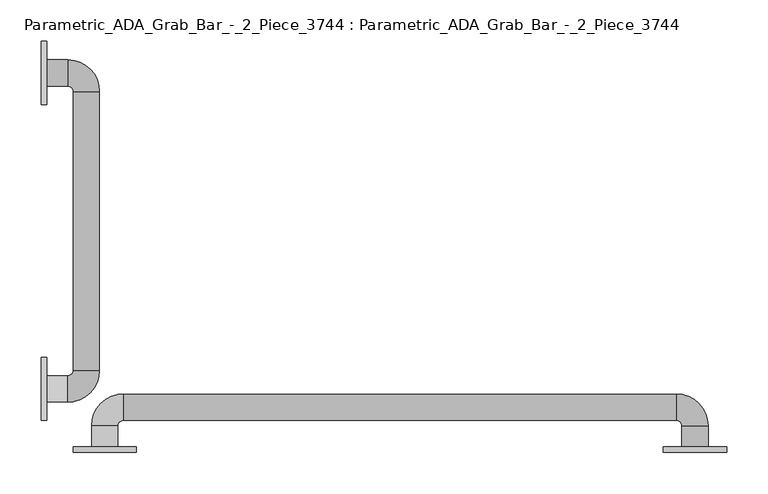
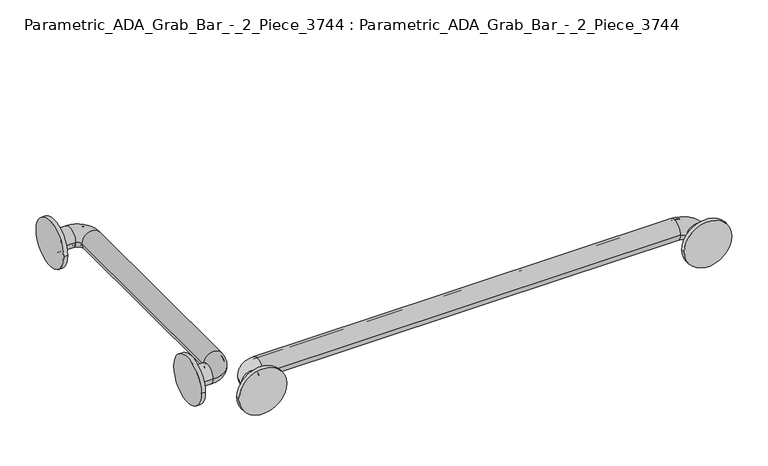
"""IFC4 building model written with IfcOpenShell, lengths in millimetres: proxy geometry, Parametric_ADA_Grab_Bar_-_2_Piece_3744 : Parametric_ADA_Grab_Bar_-_2_Piece_3744."""

from ifc_helpers import new_model, si_unit, point, frame, frame_2d, origin, place, context, project, spatial, polyline, circle_curve, ellipse_curve, trimmed, segment, composite_curve, outline, extrude, source, transform, mapped, element, save
from ifc_brep_helpers import plane_surface, cylinder_surface, revolved_surface, advanced_brep


def parametric_ada_grab_bar_2_piece_3744_parametric_ada_grab_bar_39837210(model_context):
    return source(origin(), model_context, "Body", "SolidModel", [
        advanced_brep(
        [(6.35, 454.81875, 838.2), (6.35, 486.56875, 838.2), (6.35, 457.99375, 838.2), (6.35, 483.39375, 838.2), (31.75, 454.81875, 838.2), (31.75, 486.56875, 838.2), (31.75, 457.99375, 838.2), (31.75, 483.39375, 838.2), (69.85, 448.46875, 838.2), (38.1, 448.46875, 838.2), (66.675, 448.46875, 838.2), (41.275, 448.46875, 838.2), (38.1, 111.91875, 838.2), (69.85, 111.91875, 838.2), (41.275, 111.91875, 838.2), (66.675, 111.91875, 838.2), (31.75, 73.81875, 838.2), (31.75, 105.56875, 838.2), (31.75, 76.99375, 838.2), (31.75, 102.39375, 838.2), (6.35, 105.56875, 838.2), (6.35, 73.81875, 838.2), (6.35, 102.39375, 838.2), (6.35, 76.99375, 838.2)],
        [
            (0, 1, circle_curve(frame((6.35, 470.69375, 838.2), z_axis=(-1.0, 0.0, 0.0), x_axis=(0.0, 1.0, 0.0)), 15.875)),
            (1, 0, circle_curve(frame((6.35, 470.69375, 838.2), z_axis=(-1.0, 0.0, 0.0), x_axis=(0.0, 1.0, 0.0)), 15.875)),
            (2, 3, circle_curve(frame((6.35, 470.69375, 838.2), z_axis=(1.0, 0.0, 0.0), x_axis=(0.0, 1.0, 0.0)), 12.7)),
            (3, 2, circle_curve(frame((6.35, 470.69375, 838.2), z_axis=(1.0, 0.0, 0.0), x_axis=(0.0, 1.0, 0.0)), 12.7)),
            (0, 4),
            (4, 5, circle_curve(frame((31.75, 470.69375, 838.2), z_axis=(-1.0, 0.0, 0.0), x_axis=(0.0, 1.0, 0.0)), 15.875)),
            (5, 1),
            (5, 4, circle_curve(frame((31.75, 470.69375, 838.2), z_axis=(-1.0, 0.0, 0.0), x_axis=(0.0, 1.0, 0.0)), 15.875)),
            (2, 6),
            (6, 7, circle_curve(frame((31.75, 470.69375, 838.2), z_axis=(1.0, 0.0, 0.0), x_axis=(0.0, 1.0, 0.0)), 12.7)),
            (7, 3),
            (7, 6, circle_curve(frame((31.75, 470.69375, 838.2), z_axis=(1.0, 0.0, 0.0), x_axis=(0.0, 1.0, 0.0)), 12.7)),
            (8, 5, circle_curve(frame((31.75, 448.46875, 838.2), z_axis=(0.0, 0.0, 1.0), x_axis=(0.0, 1.0, 0.0)), 38.1)),
            (4, 9, circle_curve(frame((31.75, 448.46875, 838.2), z_axis=(0.0, 0.0, -1.0), x_axis=(0.0, 1.0, 0.0)), 6.35)),
            (9, 8, circle_curve(frame((53.975, 448.46875, 838.2), z_axis=(0.0, 1.0, 0.0), x_axis=(1.0, 0.0, 0.0)), 15.875)),
            (8, 9, circle_curve(frame((53.975, 448.46875, 838.2), z_axis=(0.0, 1.0, 0.0), x_axis=(1.0, 0.0, 0.0)), 15.875)),
            (10, 7, circle_curve(frame((31.75, 448.46875, 838.2), z_axis=(0.0, 0.0, 1.0), x_axis=(0.0, 1.0, 0.0)), 34.925)),
            (6, 11, circle_curve(frame((31.75, 448.46875, 838.2), z_axis=(0.0, 0.0, -1.0), x_axis=(0.0, 1.0, 0.0)), 9.525)),
            (11, 10, circle_curve(frame((53.975, 448.46875, 838.2), z_axis=(0.0, -1.0, 0.0), x_axis=(1.0, 0.0, 0.0)), 12.7)),
            (10, 11, circle_curve(frame((53.975, 448.46875, 838.2), z_axis=(0.0, -1.0, 0.0), x_axis=(1.0, 0.0, 0.0)), 12.7)),
            (9, 12),
            (12, 13, circle_curve(frame((53.975, 111.91875, 838.2), z_axis=(0.0, 1.0, 0.0), x_axis=(1.0, 0.0, 0.0)), 15.875)),
            (13, 8),
            (13, 12, circle_curve(frame((53.975, 111.91875, 838.2), z_axis=(0.0, 1.0, 0.0), x_axis=(1.0, 0.0, 0.0)), 15.875)),
            (11, 14),
            (14, 15, circle_curve(frame((53.975, 111.91875, 838.2), z_axis=(0.0, -1.0, 0.0), x_axis=(1.0, 0.0, 0.0)), 12.7)),
            (15, 10),
            (15, 14, circle_curve(frame((53.975, 111.91875, 838.2), z_axis=(0.0, -1.0, 0.0), x_axis=(1.0, 0.0, 0.0)), 12.7)),
            (16, 13, circle_curve(frame((31.75, 111.91875, 838.2), z_axis=(0.0, 0.0, 1.0), x_axis=(1.0, 0.0, 0.0)), 38.1)),
            (12, 17, circle_curve(frame((31.75, 111.91875, 838.2), z_axis=(0.0, 0.0, -1.0), x_axis=(1.0, 0.0, 0.0)), 6.35)),
            (17, 16, circle_curve(frame((31.75, 89.69375, 838.2), z_axis=(1.0, -1.076610172186615e-12, 0.0), x_axis=(-1.076610172186615e-12, -1.0, 0.0)), 15.875)),
            (16, 17, circle_curve(frame((31.75, 89.69375, 838.2), z_axis=(1.0, 0.0, 0.0), x_axis=(0.0, -1.0, 0.0)), 15.875)),
            (18, 15, circle_curve(frame((31.75, 111.91875, 838.2), z_axis=(0.0, 0.0, 1.0), x_axis=(1.0, 0.0, 0.0)), 34.925)),
            (14, 19, circle_curve(frame((31.75, 111.91875, 838.2), z_axis=(0.0, 0.0, -1.0), x_axis=(1.0, 0.0, 0.0)), 9.525)),
            (19, 18, circle_curve(frame((31.75, 89.69375, 838.2), z_axis=(-1.0, 0.0, 0.0), x_axis=(0.0, -1.0, 0.0)), 12.7)),
            (18, 19, circle_curve(frame((31.75, 89.69375, 838.2), z_axis=(-1.0, 0.0, 0.0), x_axis=(0.0, -1.0, 0.0)), 12.7)),
            (20, 21, circle_curve(frame((6.35, 89.69375, 838.2), z_axis=(-1.0, 0.0, 0.0), x_axis=(0.0, -1.0, 0.0)), 15.875)),
            (21, 20, circle_curve(frame((6.35, 89.69375, 838.2), z_axis=(-1.0, 0.0, 0.0), x_axis=(0.0, -1.0, 0.0)), 15.875)),
            (22, 23, circle_curve(frame((6.35, 89.69375, 838.2), z_axis=(1.0, 0.0, 0.0), x_axis=(0.0, -1.0, 0.0)), 12.7)),
            (23, 22, circle_curve(frame((6.35, 89.69375, 838.2), z_axis=(1.0, 0.0, 0.0), x_axis=(0.0, -1.0, 0.0)), 12.7)),
            (17, 20),
            (21, 16),
            (19, 22),
            (23, 18),
        ],
        [
            plane_surface(frame((6.35, 470.69375, 838.2), z_axis=(-1.0, 0.0, 0.0), x_axis=(0.0, 0.0, 1.0))),
            cylinder_surface(frame((6.35, 470.69375, 838.2), z_axis=(-1.0, 0.0, 0.0), x_axis=(0.0, 1.0, 0.0)), 15.875),
            revolved_surface(polyline([(31.75, 483.39375, 838.2), (6.35, 483.39375, 838.2)]), (6.35, 470.69375, 838.2), (1.0, 0.0, 0.0)),
            revolved_surface(trimmed(ellipse_curve(frame((31.75, 470.69375, 838.2), z_axis=(-1.0, 0.0, 0.0), x_axis=(0.0, 1.0, 0.0)), 15.875, 15.875), [point((31.75, 454.81875, 838.2))], [point((31.75, 486.56875, 838.2))], True, "CARTESIAN"), (31.75, 448.46875, 838.2), (0.0, 0.0, -1.0)),
            revolved_surface(trimmed(ellipse_curve(frame((31.75, 470.69375, 838.2), z_axis=(-1.0, 0.0, 0.0), x_axis=(0.0, 1.0, 0.0)), 15.875, 15.875), [point((31.75, 486.56875, 838.2))], [point((31.75, 454.81875, 838.2))], True, "CARTESIAN"), (31.75, 448.46875, 838.2), (0.0, 0.0, -1.0)),
            revolved_surface(trimmed(ellipse_curve(frame((31.75, 470.69375, 838.2), z_axis=(1.0, 0.0, 0.0), x_axis=(0.0, 1.0, 0.0)), 12.7, 12.7), [point((31.75, 457.99375, 838.2))], [point((31.75, 483.39375, 838.2))], True, "CARTESIAN"), (31.75, 448.46875, 838.2), (0.0, 0.0, -1.0)),
            revolved_surface(trimmed(ellipse_curve(frame((31.75, 470.69375, 838.2), z_axis=(1.0, 0.0, 0.0), x_axis=(0.0, 1.0, 0.0)), 12.7, 12.7), [point((31.75, 483.39375, 838.2))], [point((31.75, 457.99375, 838.2))], True, "CARTESIAN"), (31.75, 448.46875, 838.2), (0.0, 0.0, -1.0)),
            cylinder_surface(frame((53.975, 448.46875, 838.2), z_axis=(0.0, 1.0, 0.0), x_axis=(1.0, 0.0, 0.0)), 15.875),
            revolved_surface(polyline([(66.675, 111.91874999999999, 838.2), (66.675, 448.46875, 838.2)]), (53.975, 448.46875, 838.2), (0.0, -1.0, 0.0)),
            revolved_surface(trimmed(ellipse_curve(frame((53.975, 111.91875, 838.2), z_axis=(0.0, 1.0, 0.0), x_axis=(1.0, 0.0, 0.0)), 15.875, 15.875), [point((38.1, 111.91875, 838.2))], [point((69.85, 111.91875, 838.2))], True, "CARTESIAN"), (31.75, 111.91875, 838.2), (0.0, 0.0, -1.0)),
            revolved_surface(trimmed(ellipse_curve(frame((53.975, 111.91875, 838.2), z_axis=(0.0, 1.0, 0.0), x_axis=(1.0, 0.0, 0.0)), 15.875, 15.875), [point((69.85, 111.91875, 838.2))], [point((38.1, 111.91875, 838.2))], True, "CARTESIAN"), (31.75, 111.91875, 838.2), (0.0, 0.0, -1.0)),
            revolved_surface(trimmed(ellipse_curve(frame((53.975, 111.91875, 838.2), z_axis=(0.0, -1.0, 0.0), x_axis=(1.0, 0.0, 0.0)), 12.7, 12.7), [point((41.275, 111.91875, 838.2))], [point((66.675, 111.91875, 838.2))], True, "CARTESIAN"), (31.75, 111.91875, 838.2), (0.0, 0.0, -1.0)),
            revolved_surface(trimmed(ellipse_curve(frame((53.975, 111.91875, 838.2), z_axis=(0.0, -1.0, 0.0), x_axis=(1.0, 0.0, 0.0)), 12.7, 12.7), [point((66.675, 111.91875, 838.2))], [point((41.275, 111.91875, 838.2))], True, "CARTESIAN"), (31.75, 111.91875, 838.2), (0.0, 0.0, -1.0)),
            plane_surface(frame((6.35, 89.69375, 838.2), z_axis=(-1.0, 0.0, 0.0), x_axis=(0.0, 0.0, 1.0))),
            cylinder_surface(frame((31.75, 89.69375, 838.2), z_axis=(1.0, 0.0, 0.0), x_axis=(0.0, -1.0, 0.0)), 15.875),
            revolved_surface(polyline([(6.350000000000001, 76.99374999999999, 838.2), (31.75, 76.99374999999999, 838.2)]), (31.75, 89.69375, 838.2), (-1.0, 0.0, 0.0)),
        ],
        [
            (0, [[1, 2], [3, 4]]),
            (1, [[-1, 5, 6, 7]]),
            (1, [[-2, -7, 8, -5]]),
            (2, [[-3, 9, 10, 11]]),
            (2, [[-4, -11, 12, -9]]),
            (3, [[13, -6, 14, 15]]),
            (4, [[-14, -8, -13, 16]]),
            (5, [[17, -10, 18, 19]]),
            (6, [[-18, -12, -17, 20]]),
            (7, [[-15, 21, 22, 23]]),
            (7, [[-16, -23, 24, -21]]),
            (8, [[-19, 25, 26, 27]]),
            (8, [[-20, -27, 28, -25]]),
            (9, [[29, -22, 30, 31]]),
            (10, [[-30, -24, -29, 32]]),
            (11, [[33, -26, 34, 35]]),
            (12, [[-34, -28, -33, 36]]),
            (13, [[37, 38], [39, 40]]),
            (14, [[-31, 41, -38, 42]]),
            (14, [[-32, -42, -37, -41]]),
            (15, [[-35, 43, -40, 44]]),
            (15, [[-36, -44, -39, -43]]),
        ],
    ),
        advanced_brep(
        [(92.075, 19.84375, 838.2), (60.325, 19.84375, 838.2), (88.9, 19.84375, 838.2), (63.5, 19.84375, 838.2), (92.075, 45.24375, 838.2), (60.325, 45.24375, 838.2), (88.9, 45.24375, 838.2), (63.5, 45.24375, 838.2), (98.425, 83.34375, 838.2), (98.425, 51.59375, 838.2), (98.425, 80.16875, 838.2), (98.425, 54.76875, 838.2), (765.175, 51.59375, 838.2), (765.175, 83.34375, 838.2), (765.175, 54.76875, 838.2), (765.175, 80.16875, 838.2), (803.275, 45.24375, 838.2), (771.525, 45.24375, 838.2), (800.1, 45.24375, 838.2), (774.7, 45.24375, 838.2), (771.525, 19.84375, 838.2), (803.275, 19.84375, 838.2), (774.7, 19.84375, 838.2), (800.1, 19.84375, 838.2)],
        [
            (0, 1, circle_curve(frame((76.2, 19.84375, 838.2), z_axis=(0.0, -1.0, 0.0), x_axis=(-1.0, 0.0, 0.0)), 15.875)),
            (1, 0, circle_curve(frame((76.2, 19.84375, 838.2), z_axis=(0.0, -1.0, 0.0), x_axis=(-1.0, 0.0, 0.0)), 15.875)),
            (2, 3, circle_curve(frame((76.2, 19.84375, 838.2), z_axis=(0.0, 1.0, 0.0), x_axis=(-1.0, 0.0, 0.0)), 12.7)),
            (3, 2, circle_curve(frame((76.2, 19.84375, 838.2), z_axis=(0.0, 1.0, 0.0), x_axis=(-1.0, 0.0, 0.0)), 12.7)),
            (0, 4),
            (4, 5, circle_curve(frame((76.2, 45.24375, 838.2), z_axis=(0.0, -1.0, 0.0), x_axis=(-1.0, 0.0, 0.0)), 15.875)),
            (5, 1),
            (5, 4, circle_curve(frame((76.2, 45.24375, 838.2), z_axis=(0.0, -1.0, 0.0), x_axis=(-1.0, 0.0, 0.0)), 15.875)),
            (2, 6),
            (6, 7, circle_curve(frame((76.2, 45.24375, 838.2), z_axis=(0.0, 1.0, 0.0), x_axis=(-1.0, 0.0, 0.0)), 12.7)),
            (7, 3),
            (7, 6, circle_curve(frame((76.2, 45.24375, 838.2), z_axis=(0.0, 1.0, 0.0), x_axis=(-1.0, 0.0, 0.0)), 12.7)),
            (8, 5, circle_curve(frame((98.425, 45.24375, 838.2), z_axis=(0.0, 0.0, 1.0), x_axis=(-1.0, 0.0, 0.0)), 38.1)),
            (4, 9, circle_curve(frame((98.425, 45.24375, 838.2), z_axis=(0.0, 0.0, -1.0), x_axis=(-1.0, 0.0, 0.0)), 6.35)),
            (9, 8, circle_curve(frame((98.425, 67.46875, 838.2), z_axis=(-1.0, 0.0, 0.0), x_axis=(0.0, 1.0, 0.0)), 15.875)),
            (8, 9, circle_curve(frame((98.425, 67.46875, 838.2), z_axis=(-1.0, 0.0, 0.0), x_axis=(0.0, 1.0, 0.0)), 15.875)),
            (10, 7, circle_curve(frame((98.425, 45.24375, 838.2), z_axis=(0.0, 0.0, 1.0), x_axis=(-1.0, 0.0, 0.0)), 34.925)),
            (6, 11, circle_curve(frame((98.425, 45.24375, 838.2), z_axis=(0.0, 0.0, -1.0), x_axis=(-1.0, 0.0, 0.0)), 9.525)),
            (11, 10, circle_curve(frame((98.425, 67.46875, 838.2), z_axis=(1.0, 0.0, 0.0), x_axis=(0.0, 1.0, 0.0)), 12.7)),
            (10, 11, circle_curve(frame((98.425, 67.46875, 838.2), z_axis=(1.0, 0.0, 0.0), x_axis=(0.0, 1.0, 0.0)), 12.7)),
            (9, 12),
            (12, 13, circle_curve(frame((765.175, 67.46875, 838.2), z_axis=(-1.0, 0.0, 0.0), x_axis=(0.0, 1.0, 0.0)), 15.875)),
            (13, 8),
            (13, 12, circle_curve(frame((765.175, 67.46875, 838.2), z_axis=(-1.0, 0.0, 0.0), x_axis=(0.0, 1.0, 0.0)), 15.875)),
            (11, 14),
            (14, 15, circle_curve(frame((765.175, 67.46875, 838.2), z_axis=(1.0, 0.0, 0.0), x_axis=(0.0, 1.0, 0.0)), 12.7)),
            (15, 10),
            (15, 14, circle_curve(frame((765.175, 67.46875, 838.2), z_axis=(1.0, 0.0, 0.0), x_axis=(0.0, 1.0, 0.0)), 12.7)),
            (16, 13, circle_curve(frame((765.175, 45.24375, 838.2), z_axis=(0.0, 0.0, 1.0), x_axis=(0.0, 1.0, 0.0)), 38.1)),
            (12, 17, circle_curve(frame((765.175, 45.24375, 838.2), z_axis=(0.0, 0.0, -1.0), x_axis=(0.0, 1.0, 0.0)), 6.35)),
            (17, 16, circle_curve(frame((787.4, 45.24375, 838.2), z_axis=(1.0743897261373647e-12, 1.0, 0.0), x_axis=(1.0, -1.0743897261373647e-12, 0.0)), 15.875)),
            (16, 17, circle_curve(frame((787.4, 45.24375, 838.2), z_axis=(0.0, 1.0, 0.0), x_axis=(1.0, 0.0, 0.0)), 15.875)),
            (18, 15, circle_curve(frame((765.175, 45.24375, 838.2), z_axis=(0.0, 0.0, 1.0), x_axis=(0.0, 1.0, 0.0)), 34.925)),
            (14, 19, circle_curve(frame((765.175, 45.24375, 838.2), z_axis=(0.0, 0.0, -1.0), x_axis=(0.0, 1.0, 0.0)), 9.525)),
            (19, 18, circle_curve(frame((787.4, 45.24375, 838.2), z_axis=(0.0, -1.0, 0.0), x_axis=(1.0, 0.0, 0.0)), 12.7)),
            (18, 19, circle_curve(frame((787.4, 45.24375, 838.2), z_axis=(0.0, -1.0, 0.0), x_axis=(1.0, 0.0, 0.0)), 12.7)),
            (20, 21, circle_curve(frame((787.4, 19.84375, 838.2), z_axis=(0.0, -1.0, 0.0), x_axis=(1.0, 0.0, 0.0)), 15.875)),
            (21, 20, circle_curve(frame((787.4, 19.84375, 838.2), z_axis=(0.0, -1.0, 0.0), x_axis=(1.0, 0.0, 0.0)), 15.875)),
            (22, 23, circle_curve(frame((787.4, 19.84375, 838.2), z_axis=(0.0, 1.0, 0.0), x_axis=(1.0, 0.0, 0.0)), 12.7)),
            (23, 22, circle_curve(frame((787.4, 19.84375, 838.2), z_axis=(0.0, 1.0, 0.0), x_axis=(1.0, 0.0, 0.0)), 12.7)),
            (17, 20),
            (21, 16),
            (19, 22),
            (23, 18),
        ],
        [
            plane_surface(frame((76.2, 19.84375, 838.2), z_axis=(0.0, -1.0, 0.0), x_axis=(0.0, 0.0, 1.0))),
            cylinder_surface(frame((76.2, 19.84375, 838.2), z_axis=(0.0, -1.0, 0.0), x_axis=(-1.0, 0.0, 0.0)), 15.875),
            revolved_surface(polyline([(63.5, 45.24375, 838.2), (63.5, 19.84375, 838.2)]), (76.2, 19.84375, 838.2), (0.0, 1.0, 0.0)),
            revolved_surface(trimmed(ellipse_curve(frame((76.2, 45.24375, 838.2), z_axis=(0.0, -1.0, 0.0), x_axis=(-1.0, 0.0, 0.0)), 15.875, 15.875), [point((92.075, 45.24375, 838.2))], [point((60.325, 45.24375, 838.2))], True, "CARTESIAN"), (98.425, 45.24375, 838.2), (0.0, 0.0, -1.0)),
            revolved_surface(trimmed(ellipse_curve(frame((76.2, 45.24375, 838.2), z_axis=(0.0, -1.0, 0.0), x_axis=(-1.0, 0.0, 0.0)), 15.875, 15.875), [point((60.325, 45.24375, 838.2))], [point((92.075, 45.24375, 838.2))], True, "CARTESIAN"), (98.425, 45.24375, 838.2), (0.0, 0.0, -1.0)),
            revolved_surface(trimmed(ellipse_curve(frame((76.2, 45.24375, 838.2), z_axis=(0.0, 1.0, 0.0), x_axis=(-1.0, 0.0, 0.0)), 12.7, 12.7), [point((88.9, 45.24375, 838.2))], [point((63.5, 45.24375, 838.2))], True, "CARTESIAN"), (98.425, 45.24375, 838.2), (0.0, 0.0, -1.0)),
            revolved_surface(trimmed(ellipse_curve(frame((76.2, 45.24375, 838.2), z_axis=(0.0, 1.0, 0.0), x_axis=(-1.0, 0.0, 0.0)), 12.7, 12.7), [point((63.5, 45.24375, 838.2))], [point((88.9, 45.24375, 838.2))], True, "CARTESIAN"), (98.425, 45.24375, 838.2), (0.0, 0.0, -1.0)),
            cylinder_surface(frame((98.425, 67.46875, 838.2), z_axis=(-1.0, 0.0, 0.0), x_axis=(0.0, 1.0, 0.0)), 15.875),
            revolved_surface(polyline([(765.175, 80.16875, 838.2), (98.425, 80.16875, 838.2)]), (98.425, 67.46875, 838.2), (1.0, 0.0, 0.0)),
            revolved_surface(trimmed(ellipse_curve(frame((765.175, 67.46875, 838.2), z_axis=(-1.0, 0.0, 0.0), x_axis=(0.0, 1.0, 0.0)), 15.875, 15.875), [point((765.175, 51.59375, 838.2))], [point((765.175, 83.34375, 838.2))], True, "CARTESIAN"), (765.175, 45.24375, 838.2), (0.0, 0.0, -1.0)),
            revolved_surface(trimmed(ellipse_curve(frame((765.175, 67.46875, 838.2), z_axis=(-1.0, 0.0, 0.0), x_axis=(0.0, 1.0, 0.0)), 15.875, 15.875), [point((765.175, 83.34375, 838.2))], [point((765.175, 51.59375, 838.2))], True, "CARTESIAN"), (765.175, 45.24375, 838.2), (0.0, 0.0, -1.0)),
            revolved_surface(trimmed(ellipse_curve(frame((765.175, 67.46875, 838.2), z_axis=(1.0, 0.0, 0.0), x_axis=(0.0, 1.0, 0.0)), 12.7, 12.7), [point((765.175, 54.76875, 838.2))], [point((765.175, 80.16875, 838.2))], True, "CARTESIAN"), (765.175, 45.24375, 838.2), (0.0, 0.0, -1.0)),
            revolved_surface(trimmed(ellipse_curve(frame((765.175, 67.46875, 838.2), z_axis=(1.0, 0.0, 0.0), x_axis=(0.0, 1.0, 0.0)), 12.7, 12.7), [point((765.175, 80.16875, 838.2))], [point((765.175, 54.76875, 838.2))], True, "CARTESIAN"), (765.175, 45.24375, 838.2), (0.0, 0.0, -1.0)),
            plane_surface(frame((787.4, 19.84375, 838.2), z_axis=(0.0, -1.0, 0.0), x_axis=(0.0, 0.0, 1.0))),
            cylinder_surface(frame((787.4, 45.24375, 838.2), z_axis=(0.0, 1.0, 0.0), x_axis=(1.0, 0.0, 0.0)), 15.875),
            revolved_surface(polyline([(800.1, 19.84375, 838.2), (800.1, 45.24375, 838.2)]), (787.4, 45.24375, 838.2), (0.0, -1.0, 0.0)),
        ],
        [
            (0, [[1, 2], [3, 4]]),
            (1, [[-1, 5, 6, 7]]),
            (1, [[-2, -7, 8, -5]]),
            (2, [[-3, 9, 10, 11]]),
            (2, [[-4, -11, 12, -9]]),
            (3, [[13, -6, 14, 15]]),
            (4, [[-14, -8, -13, 16]]),
            (5, [[17, -10, 18, 19]]),
            (6, [[-18, -12, -17, 20]]),
            (7, [[-15, 21, 22, 23]]),
            (7, [[-16, -23, 24, -21]]),
            (8, [[-19, 25, 26, 27]]),
            (8, [[-20, -27, 28, -25]]),
            (9, [[29, -22, 30, 31]]),
            (10, [[-30, -24, -29, 32]]),
            (11, [[33, -26, 34, 35]]),
            (12, [[-34, -28, -33, 36]]),
            (13, [[37, 38], [39, 40]]),
            (14, [[-31, 41, -38, 42]]),
            (14, [[-32, -42, -37, -41]]),
            (15, [[-35, 43, -40, 44]]),
            (15, [[-36, -44, -39, -43]]),
        ],
    ),
        extrude(outline(composite_curve([segment(trimmed(circle_curve(frame_2d((89.69375, 838.2)), 38.1), [point((51.59375, 838.2))], [point((127.79375, 838.2))], False, "CARTESIAN"), True, "CONTINUOUS"), segment(trimmed(circle_curve(frame_2d((89.69375, 838.2)), 38.1), [point((127.79375, 838.2))], [point((51.59375, 838.2))], False, "CARTESIAN"), True, "CONTINUOUS")], self_intersect=False)), frame((0.0, 0.0, 0.0), z_axis=(1.0, 0.0, 0.0), x_axis=(0.0, 1.0, 0.0)), (0.0, 0.0, 1.0), 6.35),
        extrude(outline(composite_curve([segment(trimmed(circle_curve(frame_2d((470.69375, 838.2)), 38.1), [point((432.59375, 838.2))], [point((508.79375, 838.2))], False, "CARTESIAN"), True, "CONTINUOUS"), segment(trimmed(circle_curve(frame_2d((470.69375, 838.2)), 38.1), [point((508.79375, 838.2))], [point((432.59375, 838.2))], False, "CARTESIAN"), True, "CONTINUOUS")], self_intersect=False)), frame((0.0, 0.0, 0.0), z_axis=(1.0, 0.0, 0.0), x_axis=(0.0, 1.0, 0.0)), (0.0, 0.0, 1.0), 6.35),
        extrude(outline(composite_curve([segment(trimmed(circle_curve(frame_2d((838.2, 787.4)), 38.1), [point((838.2, 749.3))], [point((838.2, 825.5))], False, "CARTESIAN"), True, "CONTINUOUS"), segment(trimmed(circle_curve(frame_2d((838.2, 787.4)), 38.1), [point((838.2, 825.5))], [point((838.2, 749.3))], False, "CARTESIAN"), True, "CONTINUOUS")], self_intersect=False)), frame((0.0, 13.49375, 0.0), z_axis=(0.0, 1.0, 0.0), x_axis=(0.0, 0.0, 1.0)), (0.0, 0.0, 1.0), 6.35),
        extrude(outline(composite_curve([segment(trimmed(circle_curve(frame_2d((838.2, 76.2)), 38.1), [point((838.2, 38.1))], [point((838.2, 114.3))], False, "CARTESIAN"), True, "CONTINUOUS"), segment(trimmed(circle_curve(frame_2d((838.2, 76.2)), 38.1), [point((838.2, 114.3))], [point((838.2, 38.1))], False, "CARTESIAN"), True, "CONTINUOUS")], self_intersect=False)), frame((0.0, 13.49375, 0.0), z_axis=(0.0, 1.0, 0.0), x_axis=(0.0, 0.0, 1.0)), (0.0, 0.0, 1.0), 6.35),
    ])


if __name__ == "__main__":
    model = new_model("IFC4")
    model_context = context("Model", 3, world=origin())
    ifc_project = project(units=[si_unit("LENGTHUNIT", "METRE", prefix="MILLI")], contexts=[model_context])
    site = spatial("IfcSite", under=ifc_project)
    building = spatial("IfcBuilding", under=site)
    placement = place(None, origin())
    parametric_ada_grab_bar_2_piece_3744_parametric_ada_grab_bar_shape = parametric_ada_grab_bar_2_piece_3744_parametric_ada_grab_bar_39837210(model_context)
    element("IfcBuildingElementProxy", 1, Name="Parametric_ADA_Grab_Bar_-_2_Piece_3744 : Parametric_ADA_Grab_Bar_-_2_Piece_3744", ObjectType="Parametric_ADA_Grab_Bar_-_2_Piece_3744 : Parametric_ADA_Grab_Bar_-_2_Piece_3744", at=placement, inside=building, context=model_context, shape_type="MappedRepresentation", body=[
        mapped(parametric_ada_grab_bar_2_piece_3744_parametric_ada_grab_bar_shape, transform((0.0, 0.0, 0.0), x_axis=(1.0, 0.0, 0.0), y_axis=(0.0, 1.0, 0.0), z_axis=(0.0, 0.0, 1.0))),
    ])
    save(model, "model.ifc")

# Revit data of these elements
# Type "Parametric_ADA_Grab_Bar_-_2_Piece_3744 : Parametric_ADA_Grab_Bar_-_2_Piece_3744"
#   Keynote = "M10281313.01"
#   Grab bar length (42" min) = 1' - 3"
#   Grab bar height = 2' - 9"
#   Grab bar Length (36" min) = 2' - 4"
#   Face of Wall to Grab bar (6" max) = 0' - 3"
#   Face of Wall to Grab bar (12" max) = 0' - 3"
# Element 1 (IfcBuildingElementProxy, "Parametric_ADA_Grab_Bar_-_2_Piece_3744 : Parametric_ADA_Grab_Bar_-_2_Piece_3744")
#   Materials on its faces: "Stainless Steel"
# Materials
#   "Stainless Steel": class "Metal", colour RGB 0 0 0, transparency 0, Description = "Stainless Steel 18/8", Cost = 0
